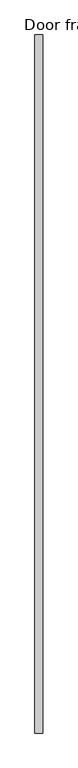
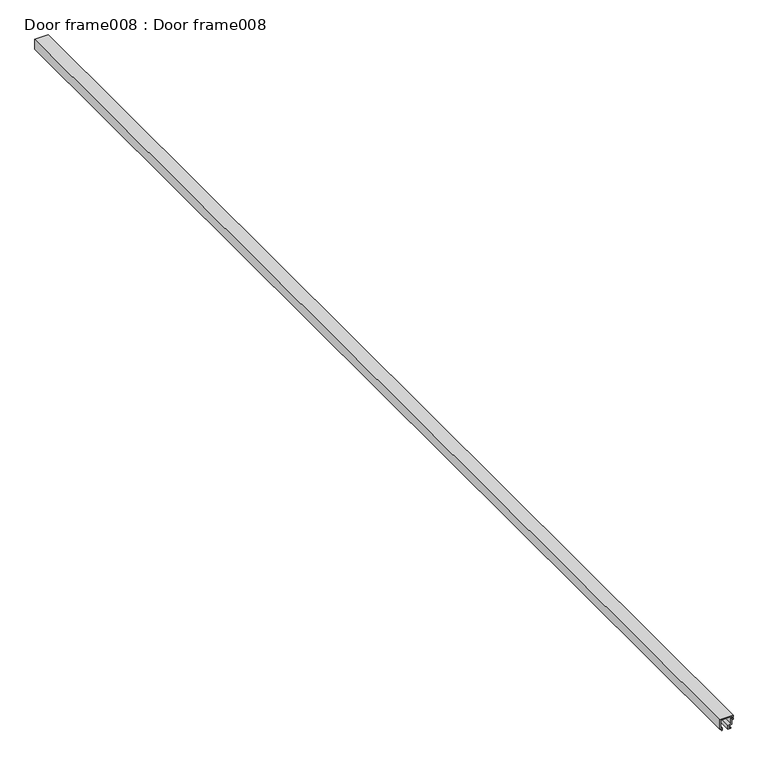
"""IFC4 building model written with IfcOpenShell, lengths in millimetres: proxy geometry, Door frame008 : Door frame008."""

from ifc_helpers import new_model, si_unit, frame, origin, place, context, project, spatial, polyline, outline, extrude, source, transform, mapped, element, save


def door_frame008_door_frame008_4371c8f4(model_context):
    return source(origin(), model_context, "Body", "SweptSolid", [
        extrude(outline(polyline([(36665.0550947, 15518.5928473), (36665.0550947, 15523.2947939), (36666.4520947, 15523.2947939), (36666.4520947, 15520.1676473), (36670.1011414, 15520.1676473), (36671.9000345, 15524.8924515), (36679.2790947, 15524.8924515), (36679.2790947, 15527.4324515), (36681.9249044, 15527.4324515), (36681.9249044, 15526.1777759), (36680.6298938, 15526.1777759), (36680.6298938, 15524.6927561), (36685.5545864, 15524.6927561), (36685.5545864, 15526.1777759), (36684.2230088, 15526.1777759), (36684.2230088, 15527.4324515), (36686.8990947, 15527.4324515), (36686.8990947, 15504.8264515), (36669.5427612, 15504.8264515), (36669.5427612, 15507.7728515), (36668.8374665, 15508.1726577), (36667.4225662, 15507.3557647), (36666.0872218, 15508.6911091), (36666.4062067, 15509.5508515), (36670.8462947, 15509.5508515), (36670.8462947, 15506.2234515), (36685.5020947, 15506.2234515), (36685.5020947, 15523.4954515), (36673.0532282, 15523.4954515), (36671.1866406, 15518.5928473), (36665.0550947, 15518.5928473)])), frame((0.0, -1052.8906567, 0.0), z_axis=(0.0, 1.0, 0.0), x_axis=(0.0, 0.0, 1.0)), (0.0, 0.0, 1.0), 1999.85),
    ])


if __name__ == "__main__":
    model = new_model("IFC4")
    model_context = context("Model", 3, world=origin())
    ifc_project = project(units=[si_unit("LENGTHUNIT", "METRE", prefix="MILLI")], contexts=[model_context])
    site = spatial("IfcSite", under=ifc_project)
    building = spatial("IfcBuilding", under=site)
    placement = place(None, origin())
    door_frame008_door_frame008_shape = door_frame008_door_frame008_4371c8f4(model_context)
    element("IfcBuildingElementProxy", 1, Name="Door frame008 : Door frame008", ObjectType="Door frame008 : Door frame008", at=placement, inside=building, context=model_context, shape_type="MappedRepresentation", body=[
        mapped(door_frame008_door_frame008_shape, transform((0.0, 0.0, 0.0), x_axis=(1.0, 0.0, 0.0), y_axis=(0.0, 1.0, 0.0), z_axis=(0.0, 0.0, 1.0))),
    ])
    save(model, "model.ifc")

# Revit data of these elements
# Type "Door frame008 : Door frame008"
#   NameOverride = "Door frame008"
# Element 1 (IfcBuildingElementProxy, "Door frame008 : Door frame008")
#   Materials on its faces: "FLEETWOOD SERIES T-3200 SINGLE SWING DOOR FRAME"
# Materials
#   "FLEETWOOD SERIES T-3200 SINGLE SWING DOOR FRAME": class "Unassigned", colour RGB 128 128 128, transparency 0, Cost = 0
